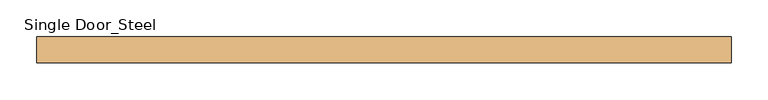
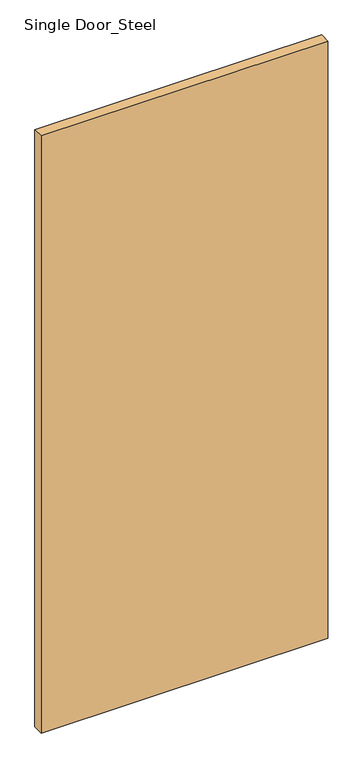
"""IFC4 building model written with IfcOpenShell, lengths in millimetres: door geometry, Single Door_Steel : H_DR_AMB_Single Door_Steel_W1000xH2100."""

from ifc_helpers import new_model, si_unit, origin, origin_with_axes, place, context, project, spatial, polyline, outline, extrude, source, transform, mapped, element, save


def single_door_steel_bf6f5e52(model_context):
    return source(origin(), model_context, "Body", "SweptSolid", [
        extrude(outline(polyline([(470.0, -130.0), (-470.0, -130.0), (-470.0, -95.0), (470.0, -95.0), (470.0, -130.0)])), origin_with_axes(), (0.0, 0.0, 1.0), 2070.0),
    ])


if __name__ == "__main__":
    model = new_model("IFC4")
    model_context = context("Model", 3, world=origin())
    ifc_project = project(units=[si_unit("LENGTHUNIT", "METRE", prefix="MILLI")], contexts=[model_context])
    site = spatial("IfcSite", under=ifc_project)
    building = spatial("IfcBuilding", under=site)
    placement = place(None, origin())
    single_door_steel_shape = single_door_steel_bf6f5e52(model_context)
    element("IfcDoor", 1, ObjectType="Single Door_Steel : H_DR_AMB_Single Door_Steel_W1000xH2100", at=placement, inside=building, context=model_context, shape_type="MappedRepresentation", body=[
        mapped(single_door_steel_shape, transform((0.0, 0.0, 0.0), x_axis=(1.0, 0.0, 0.0), y_axis=(0.0, 1.0, 0.0), z_axis=(0.0, 0.0, 1.0))),
    ])
    save(model, "model.ifc")

# Revit data of these elements
# Type "Single Door_Steel : H_DR_AMB_Single Door_Steel_W1000xH2100"
#   Type Mark = "SD"
#   Analytic Construction = "<None>"
#   프레임 투영 외부. = 25.000 mm
#   프레임 투영 내부. = 25.000 mm
#   프레임 폭 = 75.000 mm
#   Height = 2100.000 mm
#   Width = 1000.000 mm
#   Define Thermal Properties by = 1
#   문 패널 = none
#   문 프레임 = none
#   Function = (empty or 0)
#   Wall Closure = (empty or 0)
